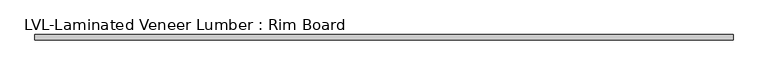
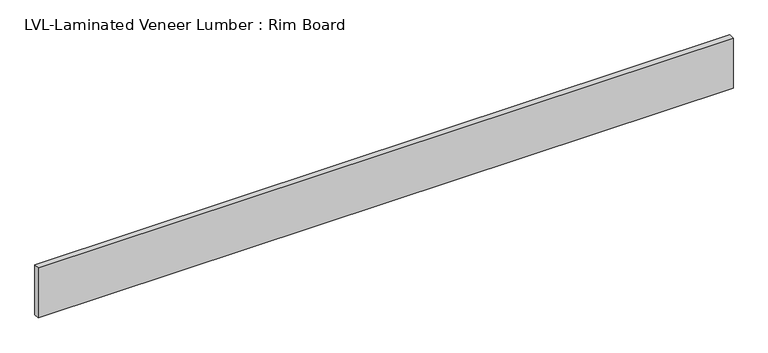
"""IFC4 building model written with IfcOpenShell, lengths in millimetres: beam geometry, LVL-Laminated Veneer Lumber : Rim Board."""

from ifc_helpers import new_model, si_unit, frame, origin, place, context, project, spatial, polyline, outline, extrude, source, transform, mapped, element, save


def lvl_laminated_veneer_lumber_rim_board_13dc89ba(model_context):
    return source(origin(), model_context, "Body", "SweptSolid", [
        extrude(outline(polyline([(1981.99375, 15.875), (1981.99375, -15.875), (-1985.16875, -15.875), (-1985.16875, 15.875), (1981.99375, 15.875)])), frame((0.0, 0.0, -150.8125), z_axis=(0.0, 0.0, 1.0), x_axis=(1.0, 0.0, 0.0)), (0.0, 0.0, 1.0), 301.625),
    ])


if __name__ == "__main__":
    model = new_model("IFC4")
    model_context = context("Model", 3, world=origin())
    ifc_project = project(units=[si_unit("LENGTHUNIT", "METRE", prefix="MILLI")], contexts=[model_context])
    site = spatial("IfcSite", under=ifc_project)
    building = spatial("IfcBuilding", under=site)
    placement = place(None, origin())
    lvl_laminated_veneer_lumber_rim_board_shape = lvl_laminated_veneer_lumber_rim_board_13dc89ba(model_context)
    element("IfcBeam", 1, ObjectType="LVL-Laminated Veneer Lumber : Rim Board", at=placement, inside=building, context=model_context, shape_type="MappedRepresentation", body=[
        mapped(lvl_laminated_veneer_lumber_rim_board_shape, transform((0.0, 0.0, 0.0), x_axis=(1.0, 0.0, 0.0), y_axis=(0.0, 1.0, 0.0), z_axis=(0.0, 0.0, 1.0))),
    ])
    save(model, "model.ifc")

# Revit data of these elements
# Type "LVL-Laminated Veneer Lumber : Rim Board"
#   Assembly Code = "B10"
#   Cost = 4.6
#   Length [instance default] = 5' - 0"
#   b = 0' - 1 1/4"
#   d = 0' - 11 7/8"
#   Structural Material [instance default] = Softwood, Lumber
# Element 1 (IfcBeam, "LVL-Laminated Veneer Lumber : Rim Board")
#   Structural Material = Douglas Fir #2
#   Materials on its faces: "Douglas Fir #2"
# Materials
#   "Softwood, Lumber": class "Wood", colour RGB 223 192 134, transparency 0, Description = "Pinus Echinata", Cost = 0
#   "Douglas Fir #2": class "Wood", colour RGB 223 192 134, transparency 0, Description = "Pinus Echinata", Cost = 0
